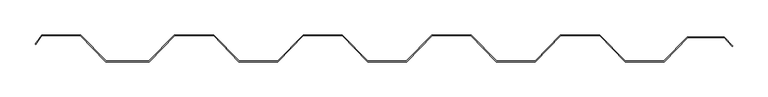
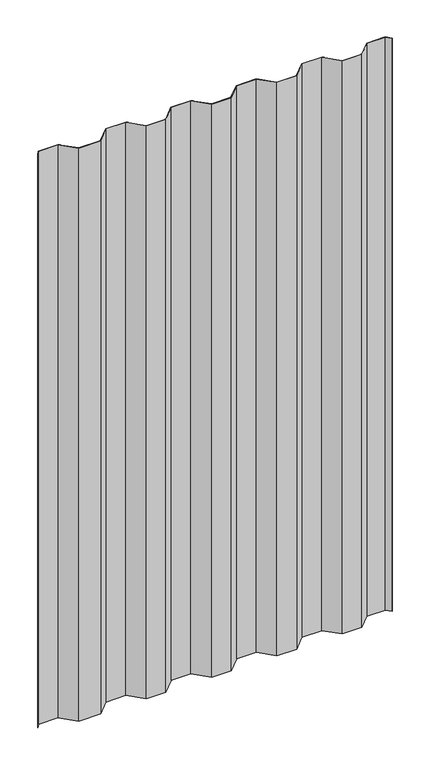
"""IFC4 building model written with IfcOpenShell, lengths in millimetres: proxy geometry, Generic Models 2:Generic Models 2:310765:Generic Models 2:310765 : Generic Models 2:Generic Models 2:310765:19 : Generic Models 2:Generic Models 2:310765:Generic Models 2:310765 : Generic Models 2:Generic Models 2:310765:300385."""

from ifc_helpers import new_model, si_unit, frame, origin, place, context, project, spatial, polyline, outline, extrude, source, transform, mapped, element, save


def generic_models_5df0ed33(model_context):
    return source(origin(), model_context, "Body", "SweptSolid", [
        extrude(outline(polyline([(570516.8090826, -578743.0895469), (570528.6648289, -578756.1976179), (570528.1028571, -578756.7595897), (570516.4567453, -578743.8832969), (570464.5503913, -578743.8832969), (570430.9184065, -578778.4413841), (570375.7388466, -578778.4413841), (570339.5766549, -578741.1351341), (570284.2015293, -578741.1351341), (570248.0393377, -578778.4413841), (570192.8588466, -578778.4413841), (570156.6966549, -578741.1351341), (570101.3215293, -578741.1351341), (570065.1593377, -578778.4413841), (570009.9788466, -578778.4413841), (569973.8166549, -578741.1351341), (569918.4415293, -578741.1351341), (569882.2793377, -578778.4413841), (569827.0988466, -578778.4413841), (569790.9366549, -578741.1351341), (569735.5615293, -578741.1351341), (569699.3993377, -578778.4413841), (569637.8688466, -578778.4413841), (569601.7066549, -578741.1351341), (569547.1780922, -578741.1351341), (569538.2367239, -578753.9047314), (569537.586522, -578753.4494551), (569546.7648921, -578740.3413841), (569602.0427005, -578740.3413841), (569638.2048921, -578777.6476341), (569699.0632921, -578777.6476341), (569735.2254838, -578740.3413841), (569791.2727005, -578740.3413841), (569827.4348921, -578777.6476341), (569881.9432921, -578777.6476341), (569918.1054838, -578740.3413841), (569974.1527005, -578740.3413841), (570010.3148921, -578777.6476341), (570064.8232921, -578777.6476341), (570100.9854838, -578740.3413841), (570157.0327005, -578740.3413841), (570193.1948921, -578777.6476341), (570247.7032921, -578777.6476341), (570283.8654838, -578740.3413841), (570339.9127005, -578740.3413841), (570376.0748921, -578777.6476341), (570430.5832921, -578777.6476341), (570464.2152769, -578743.0895469), (570516.8090826, -578743.0895469)])), frame((0.0, 0.0, 4438.4276051), z_axis=(0.0, 0.0, 1.0), x_axis=(1.0, 0.0, 0.0)), (0.0, 0.0, 1.0), 1695.6723949),
    ])


if __name__ == "__main__":
    model = new_model("IFC4")
    model_context = context("Model", 3, world=origin())
    ifc_project = project(units=[si_unit("LENGTHUNIT", "METRE", prefix="MILLI")], contexts=[model_context])
    site = spatial("IfcSite", under=ifc_project)
    building = spatial("IfcBuilding", under=site)
    placement = place(None, origin())
    generic_models_shape = generic_models_5df0ed33(model_context)
    element("IfcBuildingElementProxy", 1, Name="Generic Models 2:Generic Models 2:310765:Generic Models 2:310765 : Generic Models 2:Generic Models 2:310765:19 : Generic Models 2:Generic Models 2:310765:Generic Models 2:310765 : Generic Models 2:Generic Models 2:310765:300385", ObjectType="Generic Models 2:Generic Models 2:310765:Generic Models 2:310765 : Generic Models 2:Generic Models 2:310765:19 : Generic Models 2:Generic Models 2:310765:Generic Models 2:310765 : Generic Models 2:Generic Models 2:310765:300385", at=placement, inside=building, context=model_context, shape_type="MappedRepresentation", body=[
        mapped(generic_models_shape, transform((0.0, 0.0, 0.0), x_axis=(1.0, 0.0, 0.0), y_axis=(0.0, 1.0, 0.0), z_axis=(0.0, 0.0, 1.0))),
    ])
    save(model, "model.ifc")

# Revit data of these elements
# Type "Generic Models 2:Generic Models 2:310765:Generic Models 2:310765 : Generic Models 2:Generic Models 2:310765:19 : Generic Models 2:Generic Models 2:310765:Generic Models 2:310765 : Generic Models 2:Generic Models 2:310765:300385"
#   NameOverride = "Generic Models 2:Generic Models 2:310765:Generic Models 2:310765 : Generic Models 2:Generic Models 2:310765:300385"
#   ObjectTypeOverride = "Generic Models 2:310765 : Generic Models 2:Generic Models 2:310765"
#   Reference = "Generic Models 2"
#   Tag = "300385"
# Element 1 (IfcBuildingElementProxy, "Generic Models 2:Generic Models 2:310765:Generic Models 2:310765 : Generic Models 2:Generic Models 2:310765:19 : Generic Models 2:Generic Models 2:310765:Generic Models 2:310765 : Generic Models 2:Generic Models 2:310765:300385")
#   Materials on its faces: "VERTICAL CORRUGATED METAL PANEL - EXPOSED FASTENERS - (MBCI 7.2 PANEL)"
# Materials
#   "VERTICAL CORRUGATED METAL PANEL - EXPOSED FASTENERS - (MBCI 7.2 PANEL)": class "Generic", colour RGB 120 120 120, transparency 0, Cost = 0
